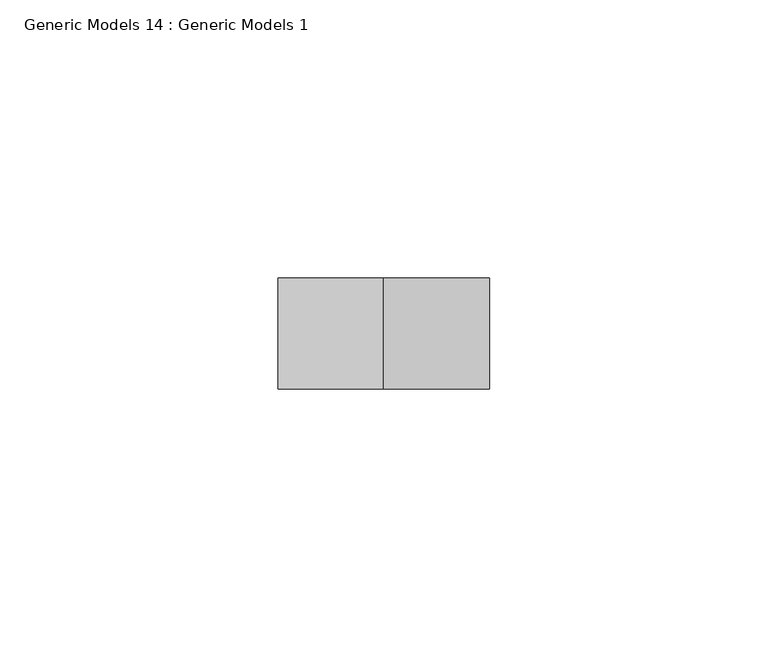
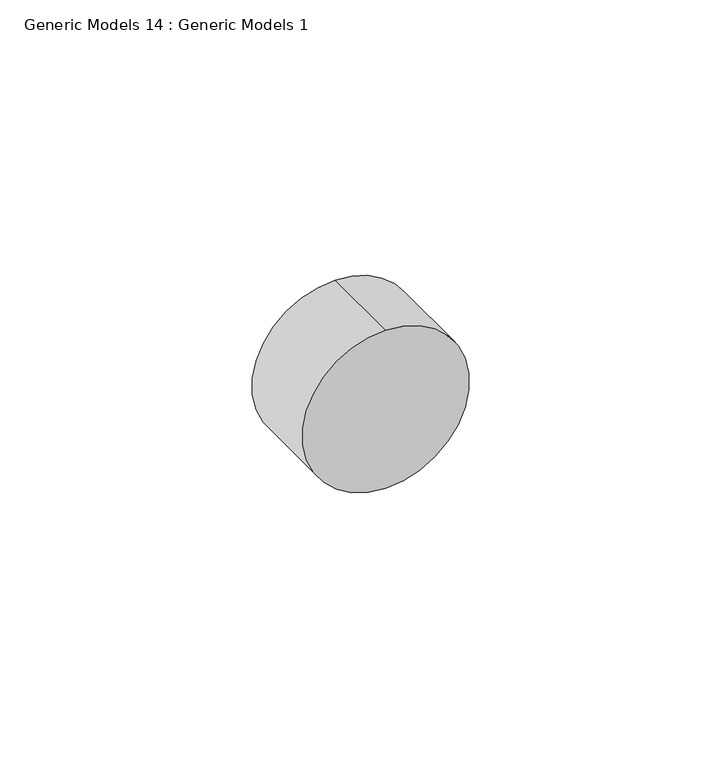
"""IFC4 building model written with IfcOpenShell, lengths in millimetres: proxy geometry, Generic Models 14 : Generic Models 1."""

import ifcopenshell
import ifcopenshell.guid

model = None  # the IFC model being written
_history = None  # IfcOwnerHistory: only IFC2X3 demands one
_inside = {}  # id of a spatial element -> (the spatial element, [elements in it])
_under = {}  # id of a project, library or spatial element -> (it, [spatial elements below it])
_declared = {}  # id of a project -> (the project, [libraries it declares])
_typed = {}  # id of a type object -> (the type object, [elements of that type])
_made_of = {}  # id of a material, layer set ... -> (it, [elements and type objects made of it])


def new_model(schema):
    """Start an empty IFC model of exactly this schema.

    Asked for "IFC4X3", IfcOpenShell would pick the latest addendum, in which some entities
    have other attributes; the version numbers below select the first issue.
    IFC2X3 requires an IfcOwnerHistory on every rooted entity: one is made here for all.
    """
    global model, _history
    if schema == "IFC4X3":
        model = ifcopenshell.file(schema_version=(4, 3, 0, 0))
    else:
        model = ifcopenshell.file(schema=schema)
    _inside.clear()
    _under.clear()
    _declared.clear()
    _typed.clear()
    _made_of.clear()
    _history = None
    if model.schema == "IFC2X3":
        org = make("IfcOrganization", Name="unknown")
        user = make(
            "IfcPersonAndOrganization",
            ThePerson=make("IfcPerson", FamilyName="unknown"),
            TheOrganization=org,
        )
        app = make(
            "IfcApplication",
            ApplicationDeveloper=org,
            Version="unknown",
            ApplicationFullName="unknown",
            ApplicationIdentifier="unknown",
        )
        _history = make(
            "IfcOwnerHistory",
            OwningUser=user,
            OwningApplication=app,
            ChangeAction="ADDED",
            CreationDate=0,
        )
    return model


def make(cls, **values):
    """One entity of the class cls with the attributes given. An attribute that is None is left unset."""
    return model.create_entity(
        cls, **{name: value for name, value in values.items() if value is not None}
    )


def rooted(cls, **values):
    """An entity with a GlobalId (a new one), such as an element, a storey or a relation."""
    return make(cls, GlobalId=ifcopenshell.guid.new(), OwnerHistory=_history, **values)


def si_unit(unit_type, name, prefix=None):
    """IfcSIUnit, for example si_unit("LENGTHUNIT", "METRE", prefix="MILLI")."""
    return make("IfcSIUnit", UnitType=unit_type, Prefix=prefix, Name=name)


def assignment(units):
    """IfcUnitAssignment: the units of a project."""
    return None if units is None else make("IfcUnitAssignment", Units=units)


def point(xyz):
    """IfcCartesianPoint."""
    return None if xyz is None else make("IfcCartesianPoint", Coordinates=xyz)


def direction(xyz):
    """IfcDirection."""
    return None if xyz is None else make("IfcDirection", DirectionRatios=xyz)


def frame(location, z_axis=None, x_axis=None):
    """IfcAxis2Placement3D, a coordinate frame: its origin and axes. An axis left out is left unset."""
    return make(
        "IfcAxis2Placement3D",
        Location=point(location),
        Axis=direction(z_axis),
        RefDirection=direction(x_axis),
    )


def frame_2d(location, x_axis=None):
    """IfcAxis2Placement2D, a coordinate frame in the plane: its origin and x axis."""
    return make(
        "IfcAxis2Placement2D", Location=point(location), RefDirection=direction(x_axis)
    )


def origin():
    """The frame at (0, 0, 0) with its axes left unset."""
    return frame((0.0, 0.0, 0.0))


def place(relative_to, where):
    """IfcLocalPlacement: puts the frame where relative to a parent placement (None: the world)."""
    return make(
        "IfcLocalPlacement", PlacementRelTo=relative_to, RelativePlacement=where
    )


def context(
    kind, dimensions, precision=None, world=None, true_north=None, identifier=None
):
    """IfcGeometricRepresentationContext, for example the 3D "Model" context."""
    return make(
        "IfcGeometricRepresentationContext",
        ContextIdentifier=identifier,
        ContextType=kind,
        CoordinateSpaceDimension=dimensions,
        Precision=precision,
        WorldCoordinateSystem=world,
        TrueNorth=true_north,
    )


def project(units=None, contexts=None):
    """IfcProject with its units and contexts."""
    return rooted(
        "IfcProject",
        Name="project",
        RepresentationContexts=contexts,
        UnitsInContext=assignment(units),
    )


def spatial(cls, under=None, at=None, **own):
    """A site, building, storey or space (cls), placed at a placement, below another one or the project."""
    s = rooted(cls, ObjectPlacement=at, **own)
    if under is not None:
        _under.setdefault(under.id(), (under, []))[1].append(s)
    return s


def circle_curve(where, radius):
    """IfcCircle in the frame where."""
    return make("IfcCircle", Position=where, Radius=radius)


def trimmed(basis, trim1, trim2, sense, master):
    """IfcTrimmedCurve: the piece of a basis curve between two trims."""
    return make(
        "IfcTrimmedCurve",
        BasisCurve=basis,
        Trim1=trim1,
        Trim2=trim2,
        SenseAgreement=sense,
        MasterRepresentation=master,
    )


def segment(curve, same_sense, transition):
    """IfcCompositeCurveSegment."""
    return make(
        "IfcCompositeCurveSegment",
        Transition=transition,
        SameSense=same_sense,
        ParentCurve=curve,
    )


def composite_curve(segments, self_intersect=None):
    """IfcCompositeCurve: segments joined end to end."""
    return make("IfcCompositeCurve", Segments=segments, SelfIntersect=self_intersect)


def outline(outer, holes=None, kind="AREA"):
    """IfcArbitraryClosedProfileDef: a profile drawn as a closed curve; with holes, ...WithVoids."""
    if holes is None:
        return make("IfcArbitraryClosedProfileDef", ProfileType=kind, OuterCurve=outer)
    return make(
        "IfcArbitraryProfileDefWithVoids",
        ProfileType=kind,
        OuterCurve=outer,
        InnerCurves=holes,
    )


def extrude(swept, where, along, depth):
    """IfcExtrudedAreaSolid: the profile swept, set in the frame where, extruded along a direction by depth."""
    return make(
        "IfcExtrudedAreaSolid",
        SweptArea=swept,
        Position=where,
        ExtrudedDirection=direction(along),
        Depth=depth,
    )


def shape(context_of_items, identifier, shape_type, items):
    """IfcShapeRepresentation: the items that make up one representation, for example the "Body"."""
    return make(
        "IfcShapeRepresentation",
        ContextOfItems=context_of_items,
        RepresentationIdentifier=identifier,
        RepresentationType=shape_type,
        Items=items,
    )


def source(mapping_origin, context_of_items, identifier, shape_type, items):
    """IfcRepresentationMap: a shape defined once, which mapped items show again and again."""
    return make(
        "IfcRepresentationMap",
        MappingOrigin=mapping_origin,
        MappedRepresentation=shape(context_of_items, identifier, shape_type, items),
    )


def transform(
    local_origin,
    x_axis=None,
    y_axis=None,
    z_axis=None,
    scale=None,
    scale2=None,
    scale3=None,
    uniform=True,
):
    """IfcCartesianTransformationOperator3D, or its non-uniform kind. x_axis, y_axis, z_axis: its Axis1, 2, 3."""
    if uniform:
        return make(
            "IfcCartesianTransformationOperator3D",
            Axis1=direction(x_axis),
            Axis2=direction(y_axis),
            LocalOrigin=point(local_origin),
            Scale=scale,
            Axis3=direction(z_axis),
        )
    return make(
        "IfcCartesianTransformationOperator3DnonUniform",
        Axis1=direction(x_axis),
        Axis2=direction(y_axis),
        LocalOrigin=point(local_origin),
        Scale=scale,
        Axis3=direction(z_axis),
        Scale2=scale2,
        Scale3=scale3,
    )


def mapped(mapping_source, mapping_target):
    """IfcMappedItem: shows the shape of a source again, moved by a transform."""
    return make(
        "IfcMappedItem", MappingSource=mapping_source, MappingTarget=mapping_target
    )


def made_of(thing, what):
    """Note that an element or type object is made of a material, layer set ...; save() writes the relation."""
    if what is not None:
        _made_of.setdefault(what.id(), (what, []))[1].append(thing)
    return thing


def element(
    cls,
    number,
    at=None,
    inside=None,
    cuts=None,
    type_object=None,
    material=None,
    context=None,
    identifier="Body",
    shape_type=None,
    held_by="IfcProductDefinitionShape",
    body=None,
    shapes=None,
    **own,
):
    """One element of the class cls, such as IfcWall. Its Tag is "e" and its number.

    at: its placement. inside: the storey or other place that contains it. cuts: it is an
    opening in that element (IfcRelVoidsElement). A single representation is given by context,
    identifier, shape_type and body (its items); several are given by shapes. held_by: the class
    of the entity that holds the representations. save() writes the other relations.
    """
    e = rooted(cls, Tag="e%d" % number, ObjectPlacement=at, **own)
    if body is not None:
        shapes = [shape(context, identifier, shape_type, body)]
    if shapes is not None:
        e.Representation = make(held_by, Representations=shapes)
    if inside is not None:
        _inside.setdefault(inside.id(), (inside, []))[1].append(e)
    if cuts is not None:
        rooted(
            "IfcRelVoidsElement", RelatingBuildingElement=cuts, RelatedOpeningElement=e
        )
    if type_object is not None:
        _typed.setdefault(type_object.id(), (type_object, []))[1].append(e)
    return made_of(e, material)


def aggregate(whole, parts):
    """IfcRelAggregates: a whole, such as a stair, and the parts it consists of."""
    return rooted("IfcRelAggregates", RelatingObject=whole, RelatedObjects=parts)


def save(model, path):
    """Write the relations noted so far, then the file.

    IfcRelAggregates (storeys below a building ...), IfcRelContainedInSpatialStructure (elements
    in a storey), IfcRelDefinesByType, IfcRelAssociatesMaterial and IfcRelDeclares: one each for
    every whole, place, type object, material and project.
    """
    for whole, parts in _under.values():
        aggregate(whole, parts)
    for where, things in _inside.values():
        rooted(
            "IfcRelContainedInSpatialStructure",
            RelatedElements=things,
            RelatingStructure=where,
        )
    for kind, things in _typed.values():
        rooted("IfcRelDefinesByType", RelatedObjects=things, RelatingType=kind)
    for what, things in _made_of.values():
        rooted("IfcRelAssociatesMaterial", RelatedObjects=things, RelatingMaterial=what)
    for by, libraries in _declared.values():
        rooted("IfcRelDeclares", RelatingContext=by, RelatedDefinitions=libraries)
    model.write(path)


def generic_models_14_generic_models_1_482cc507(model_context):
    return source(origin(), model_context, "Body", "SweptSolid", [
        extrude(outline(composite_curve([segment(trimmed(circle_curve(frame_2d((39943.2190778, 10206.2283642)), 19.1), [point((39924.1190778, 10206.2283642))], [point((39962.3190778, 10206.2283642))], False, "CARTESIAN"), True, "CONTINUOUS"), segment(trimmed(circle_curve(frame_2d((39943.2190778, 10206.2283642)), 19.1), [point((39962.3190778, 10206.2283642))], [point((39924.1190778, 10206.2283642))], False, "CARTESIAN"), True, "CONTINUOUS")], self_intersect=False)), frame((0.0, 2006.3413727, 0.0), z_axis=(0.0, 1.0, 0.0), x_axis=(0.0, 0.0, 1.0)), (0.0, 0.0, 1.0), 19.9567516),
    ])


if __name__ == "__main__":
    model = new_model("IFC4")
    model_context = context("Model", 3, world=origin())
    ifc_project = project(units=[si_unit("LENGTHUNIT", "METRE", prefix="MILLI")], contexts=[model_context])
    site = spatial("IfcSite", under=ifc_project)
    building = spatial("IfcBuilding", under=site)
    placement = place(None, origin())
    generic_models_14_generic_models_1_shape = generic_models_14_generic_models_1_482cc507(model_context)
    element("IfcBuildingElementProxy", 1, Name="Generic Models 14 : Generic Models 1", ObjectType="Generic Models 14 : Generic Models 1", at=placement, inside=building, context=model_context, shape_type="MappedRepresentation", body=[
        mapped(generic_models_14_generic_models_1_shape, transform((0.0, 0.0, 0.0), x_axis=(1.0, 0.0, 0.0), y_axis=(0.0, 1.0, 0.0), z_axis=(0.0, 0.0, 1.0))),
    ])
    save(model, "model.ifc")
